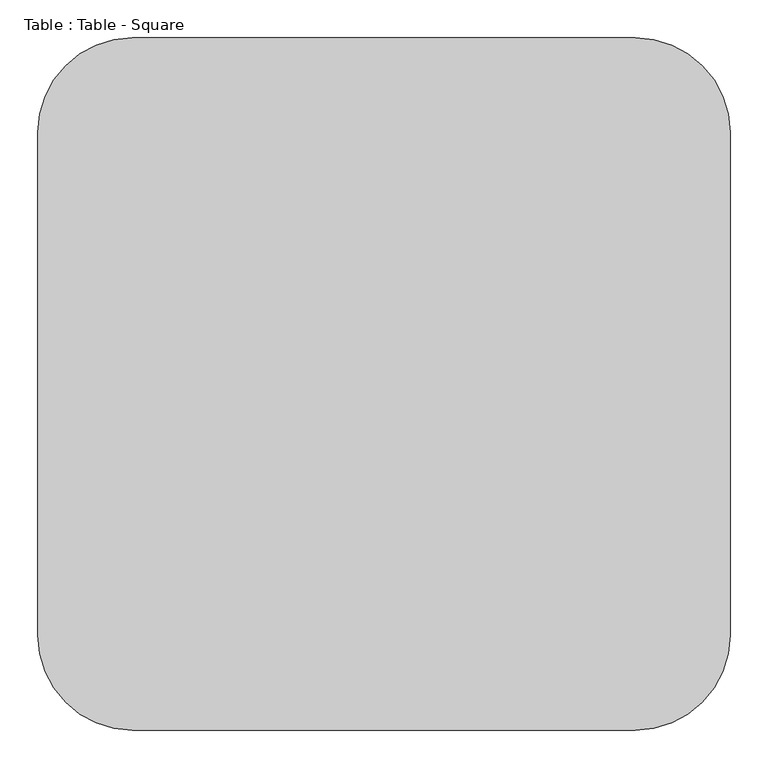
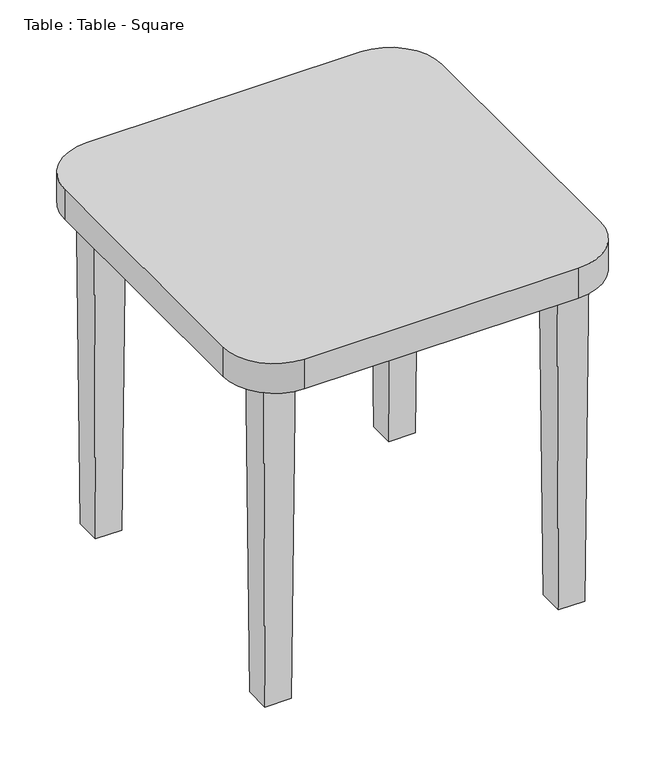
"""IFC4 building model written with IfcOpenShell, lengths in millimetres: proxy geometry, Table : Table - Square."""

from ifc_helpers import new_model, si_unit, point, frame, frame_2d, origin, place, context, project, spatial, polyline, circle_curve, trimmed, segment, composite_curve, outline, extrude, faceted_brep, source, transform, mapped, element, save


def table_table_square_807f014a(model_context):
    return source(origin(), model_context, "Body", "SolidModel", [
        faceted_brep([(-317.5, -317.5, 838.2), (-393.7, -317.5, 838.2), (-393.7, -393.7, 838.2), (-317.5, -393.7, 838.2), (-323.85, -323.85, 0.0), (-323.85, -387.35, 0.0), (-387.35, -387.35, 0.0), (-387.35, -323.85, 0.0)], [[[0, 1, 2, 3]], [[4, 5, 6, 7]], [[4, 7, 1, 0]], [[7, 6, 2, 1]], [[6, 5, 3, 2]], [[5, 4, 0, 3]]]),
        faceted_brep([(393.7, -317.5, 838.2), (317.5, -317.5, 838.2), (317.5, -393.7, 838.2), (393.7, -393.7, 838.2), (387.35, -323.85, 0.0), (387.35, -387.35, 0.0), (323.85, -387.35, 0.0), (323.85, -323.85, 0.0)], [[[0, 1, 2, 3]], [[4, 5, 6, 7]], [[4, 7, 1, 0]], [[7, 6, 2, 1]], [[6, 5, 3, 2]], [[5, 4, 0, 3]]]),
        faceted_brep([(393.7, 393.7, 838.2), (317.5, 393.7, 838.2), (317.5, 317.5, 838.2), (393.7, 317.5, 838.2), (387.35, 387.35, 0.0), (387.35, 323.85, 0.0), (323.85, 323.85, 0.0), (323.85, 387.35, 0.0)], [[[0, 1, 2, 3]], [[4, 5, 6, 7]], [[4, 7, 1, 0]], [[7, 6, 2, 1]], [[6, 5, 3, 2]], [[5, 4, 0, 3]]]),
        faceted_brep([(-317.5, 393.7, 838.2), (-393.7, 393.7, 838.2), (-393.7, 317.5, 838.2), (-317.5, 317.5, 838.2), (-323.85, 387.35, 0.0), (-323.85, 323.85, 0.0), (-387.35, 323.85, 0.0), (-387.35, 387.35, 0.0)], [[[0, 1, 2, 3]], [[4, 5, 6, 7]], [[4, 7, 1, 0]], [[7, 6, 2, 1]], [[6, 5, 3, 2]], [[5, 4, 0, 3]]]),
        extrude(outline(composite_curve([segment(trimmed(circle_curve(frame_2d((332.232, 332.232)), 124.968), [point((332.232, 457.2))], [point((457.2, 332.232))], False, "CARTESIAN"), True, "CONTINUOUS"), segment(polyline([(457.2, 332.232), (457.2, -332.232)]), True, "CONTINUOUS"), segment(trimmed(circle_curve(frame_2d((332.232, -332.232)), 124.968), [point((457.2, -332.232))], [point((332.232, -457.2))], False, "CARTESIAN"), True, "CONTINUOUS"), segment(polyline([(332.232, -457.2), (-332.232, -457.2)]), True, "CONTINUOUS"), segment(trimmed(circle_curve(frame_2d((-332.232, -332.232)), 124.968), [point((-332.232, -457.2))], [point((-457.2, -332.232))], False, "CARTESIAN"), True, "CONTINUOUS"), segment(polyline([(-457.2, -332.232), (-457.2, 332.232)]), True, "CONTINUOUS"), segment(trimmed(circle_curve(frame_2d((-332.232, 332.232)), 124.968), [point((-457.2, 332.232))], [point((-332.232, 457.2))], False, "CARTESIAN"), True, "CONTINUOUS"), segment(polyline([(-332.232, 457.2), (332.232, 457.2)]), True, "CONTINUOUS")], self_intersect=False)), frame((0.0, 0.0, 838.2), z_axis=(0.0, 0.0, 1.0), x_axis=(1.0, 0.0, 0.0)), (0.0, 0.0, 1.0), 76.2),
    ])


if __name__ == "__main__":
    model = new_model("IFC4")
    model_context = context("Model", 3, world=origin())
    ifc_project = project(units=[si_unit("LENGTHUNIT", "METRE", prefix="MILLI")], contexts=[model_context])
    site = spatial("IfcSite", under=ifc_project)
    building = spatial("IfcBuilding", under=site)
    placement = place(None, origin())
    table_table_square_shape = table_table_square_807f014a(model_context)
    element("IfcBuildingElementProxy", 1, Name="Table : Table - Square", ObjectType="Table : Table - Square", at=placement, inside=building, context=model_context, shape_type="MappedRepresentation", body=[
        mapped(table_table_square_shape, transform((0.0, 0.0, 0.0), x_axis=(1.0, 0.0, 0.0), y_axis=(0.0, 1.0, 0.0), z_axis=(0.0, 0.0, 1.0))),
    ])
    save(model, "model.ifc")

# Revit data of these elements
# Project information
#   Project Issue Date = "Issue Date"
#   Project Status = "Project Status"
#   Client Name = "Owner"
#   Project Address = "Enter address here"
#   Project Name = "Project Name"
#   Project Number = "Project Number"
# Type "Table : Table - Square"
#   Thickness [instance default] = 0' - 2"
#   Sides [instance default] = 3' - 0"
#   Leg Inset [instance default] = 0' - 4"
#   Leg Height [instance default] = 5' - 8"
#   Height [instance default] = 5' - 10"
#   Corner Fillet [instance default] = 0' - 4"
#   Default Elevation = 0
# Element 1 (IfcBuildingElementProxy, "Table : Table - Square")
#   Thickness = 0' - 3"
#   Leg Height = 2' - 9"
#   Height = 3' - 0"
#   Corner Fillet = 0' - 4.92"
